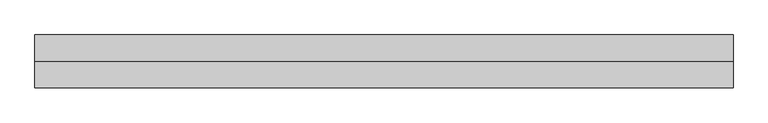
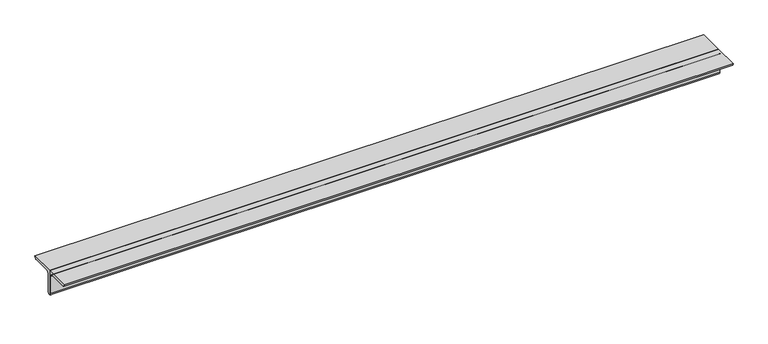
"""IFC4 building model written with IfcOpenShell, lengths in millimetres: member geometry, 0123_Steel Framing_2Ls-KSD3502 : H_SB_AR_S03_2Ls-130x130x12_HBR4."""

from ifc_helpers import new_model, si_unit, point, frame, frame_2d, origin, place, context, project, spatial, polyline, circle_curve, trimmed, segment, composite_curve, outline, extrude, source, transform, mapped, element, save


def member_9e88965d(model_context):
    return source(origin(), model_context, "Body", "SweptSolid", [
        extrude(outline(composite_curve([segment(polyline([(0.0, 36.4), (130.0, 36.4)]), True, "CONTINUOUS"), segment(trimmed(circle_curve(frame_2d((118.0, 36.4)), 12.0), [point((130.0, 36.4))], [point((118.0, 24.4))], False, "CARTESIAN"), True, "CONTINUOUS"), segment(polyline([(118.0, 24.4), (24.0, 24.4)]), True, "CONTINUOUS"), segment(trimmed(circle_curve(frame_2d((24.0, 12.4)), 12.0), [point((24.0, 24.4))], [point((12.0, 12.4))], True, "CARTESIAN"), True, "CONTINUOUS"), segment(polyline([(12.0, 12.4), (12.0, -81.6)]), True, "CONTINUOUS"), segment(trimmed(circle_curve(frame_2d((0.0, -81.6)), 12.0), [point((12.0, -81.6))], [point((0.0, -93.6))], False, "CARTESIAN"), True, "CONTINUOUS"), segment(polyline([(0.0, -93.6), (0.0, 36.4)]), True, "CONTINUOUS")], self_intersect=False)), frame((-1720.2330278, 0.0, 0.0), z_axis=(1.0, 0.0, 0.0), x_axis=(0.0, 1.0, 0.0)), (0.0, 0.0, 1.0), 3440.4660555),
        extrude(outline(composite_curve([segment(polyline([(0.0, 36.4), (0.0, -93.6)]), True, "CONTINUOUS"), segment(trimmed(circle_curve(frame_2d((0.0, -81.6)), 12.0), [point((0.0, -93.6))], [point((-12.0, -81.6))], False, "CARTESIAN"), True, "CONTINUOUS"), segment(polyline([(-12.0, -81.6), (-12.0, 12.4)]), True, "CONTINUOUS"), segment(trimmed(circle_curve(frame_2d((-24.0, 12.4)), 12.0), [point((-12.0, 12.4))], [point((-24.0, 24.4))], True, "CARTESIAN"), True, "CONTINUOUS"), segment(polyline([(-24.0, 24.4), (-118.0, 24.4)]), True, "CONTINUOUS"), segment(trimmed(circle_curve(frame_2d((-118.0, 36.4)), 12.0), [point((-118.0, 24.4))], [point((-130.0, 36.4))], False, "CARTESIAN"), True, "CONTINUOUS"), segment(polyline([(-130.0, 36.4), (0.0, 36.4)]), True, "CONTINUOUS")], self_intersect=False)), frame((-1720.2330278, 0.0, 0.0), z_axis=(1.0, 0.0, 0.0), x_axis=(0.0, 1.0, 0.0)), (0.0, 0.0, 1.0), 3440.4660555),
    ])


if __name__ == "__main__":
    model = new_model("IFC4")
    model_context = context("Model", 3, world=origin())
    ifc_project = project(units=[si_unit("LENGTHUNIT", "METRE", prefix="MILLI")], contexts=[model_context])
    site = spatial("IfcSite", under=ifc_project)
    building = spatial("IfcBuilding", under=site)
    placement = place(None, origin())
    member_shape = member_9e88965d(model_context)
    element("IfcMember", 1, ObjectType="0123_Steel Framing_2Ls-KSD3502 : H_SB_AR_S03_2Ls-130x130x12_HBR4", at=placement, inside=building, context=model_context, shape_type="MappedRepresentation", body=[
        mapped(member_shape, transform((0.0, 0.0, 0.0), x_axis=(1.0, 0.0, 0.0), y_axis=(0.0, 1.0, 0.0), z_axis=(0.0, 0.0, 1.0))),
    ])
    save(model, "model.ifc")

# Revit data of these elements
# Type "0123_Steel Framing_2Ls-KSD3502 : H_SB_AR_S03_2Ls-130x130x12_HBR4"
#   Type Mark = "HBR4"
#   Assembly Code = "B10"
#   Legs = "SLBB"
#   W = 8.97
#   Perimeter = 1.04 m²/m
#   Nominal Weight = 46.80 kgf/m
#   Length [instance default] = 1000 mm
#   Space = 0 mm
#   b = 130 mm
#   d = 130 mm
#   t = 12 mm
#   y = 36.4 mm
#   A = 0.005952 m²
#   Structural Material [instance default] = Steel ASTM A36
# Element 1 (IfcMember, "0123_Steel Framing_2Ls-KSD3502 : H_SB_AR_S03_2Ls-130x130x12_HBR4")
#   Materials on its faces: "Steel ASTM A36"
# Materials
#   "Steel ASTM A36": class "Metal", colour RGB 199 199 199, transparency 0, Description = "Structural steel, ASTM A36 Grade B, mill finish", Cost = 0
